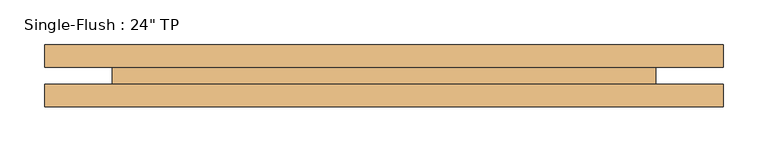
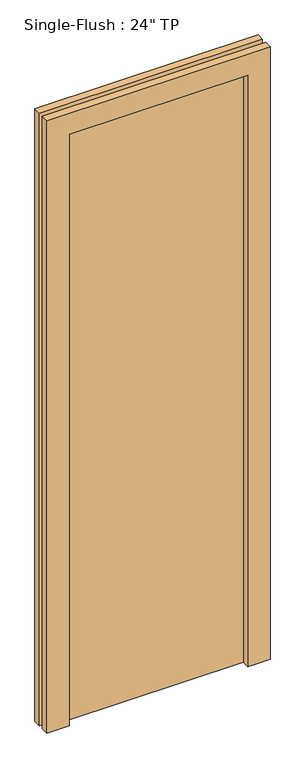
"""IFC4 building model written with IfcOpenShell, lengths in millimetres: door geometry."""

from ifc_helpers import new_model, si_unit, frame, origin, origin_with_axes, place, context, project, spatial, polyline, outline, extrude, source, transform, mapped, element, save


def door_4755addd(model_context):
    return source(origin(), model_context, "Body", "SweptSolid", [
        extrude(outline(polyline([(2209.8, -381.0), (0.0, -381.0), (0.0, -304.8), (2133.6, -304.8), (2133.6, 304.8), (0.0, 304.8), (0.0, 381.0), (2209.8, 381.0), (2209.8, -381.0)])), frame((0.0, -34.925, 0.0), z_axis=(0.0, 1.0, 0.0), x_axis=(0.0, 0.0, 1.0)), (0.0, 0.0, 1.0), 25.4),
        extrude(outline(polyline([(2209.8, 381.0), (2209.8, -381.0), (0.0, -381.0), (0.0, -304.8), (2133.6, -304.8), (2133.6, 304.8), (0.0, 304.8), (0.0, 381.0), (2209.8, 381.0)])), frame((0.0, 9.525, 0.0), z_axis=(0.0, 1.0, 0.0), x_axis=(0.0, 0.0, 1.0)), (0.0, 0.0, 1.0), 25.4),
        extrude(outline(polyline([(304.8, 9.525), (304.8, -9.525), (-304.8, -9.525), (-304.8, 9.525), (304.8, 9.525)])), origin_with_axes(), (0.0, 0.0, 1.0), 2133.6),
    ])


if __name__ == "__main__":
    model = new_model("IFC4")
    model_context = context("Model", 3, world=origin())
    ifc_project = project(units=[si_unit("LENGTHUNIT", "METRE", prefix="MILLI")], contexts=[model_context])
    site = spatial("IfcSite", under=ifc_project)
    building = spatial("IfcBuilding", under=site)
    placement = place(None, origin())
    door_shape = door_4755addd(model_context)
    element("IfcDoor", 1, ObjectType="Single-Flush : 24\" TP", at=placement, inside=building, context=model_context, shape_type="MappedRepresentation", body=[
        mapped(door_shape, transform((0.0, 0.0, 0.0), x_axis=(1.0, 0.0, 0.0), y_axis=(0.0, 1.0, 0.0), z_axis=(0.0, 0.0, 1.0))),
    ])
    save(model, "model.ifc")

# Revit data of these elements
# Type "Single-Flush : 24\" TP"
#   Type Mark = "59"
#   Construction Type Id = "MDOOR"
#   Assembly Code = "C1020"
#   Analytic Construction = "Metal"
#   Thickness = 0' - 0 3/4"
#   Heat Transfer Coefficient (U) = 3.7021 W/(m²·K)
#   Height = 7' - 0"
#   Trim Projection Ext = 0' - 1"
#   Trim Projection Int = 0' - 1"
#   Trim Width = 0' - 3"
#   Width = 2' - 0"
#   Door Material = Door - Panel
#   Frame Material = Door - Frame
#   Visual Light Transmittance = 0
#   Solar Heat Gain Coefficient = 0
#   Function = (empty or 0)
#   Wall Closure = (empty or 0)
# Element 1 (IfcDoor, "Single-Flush : 24\" TP")
#   Materials on its faces: "Door - Frame", "Door - Panel"
# Materials
#   "Door - Panel": class "Wood", colour RGB 210 159 95, transparency 0
#   "Door - Frame": class "Miscellaneous", colour RGB 118 70 51, transparency 0
